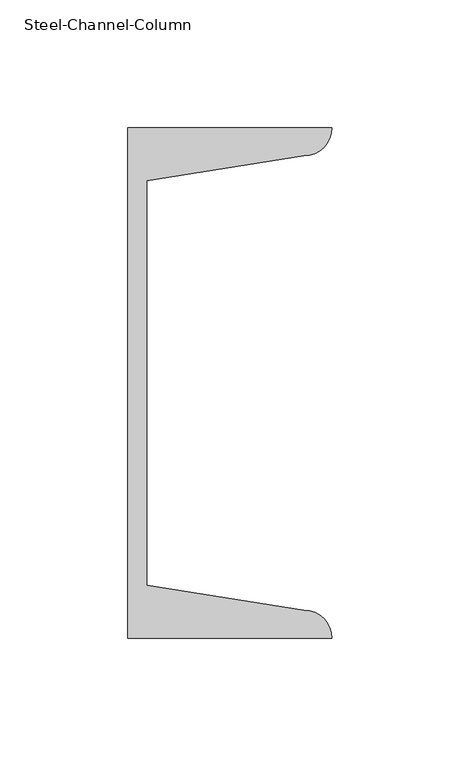
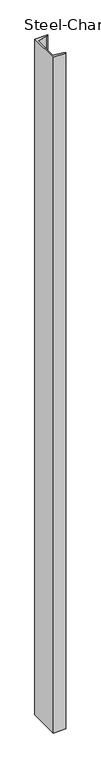
"""IFC4 building model written with IfcOpenShell, lengths in millimetres: column geometry, Steel-Channel-Column : CL126_C-200×80x7.5x11."""

import ifcopenshell
import ifcopenshell.guid

model = None  # the IFC model being written
_history = None  # IfcOwnerHistory: only IFC2X3 demands one
_inside = {}  # id of a spatial element -> (the spatial element, [elements in it])
_under = {}  # id of a project, library or spatial element -> (it, [spatial elements below it])
_declared = {}  # id of a project -> (the project, [libraries it declares])
_typed = {}  # id of a type object -> (the type object, [elements of that type])
_made_of = {}  # id of a material, layer set ... -> (it, [elements and type objects made of it])


def new_model(schema):
    """Start an empty IFC model of exactly this schema.

    Asked for "IFC4X3", IfcOpenShell would pick the latest addendum, in which some entities
    have other attributes; the version numbers below select the first issue.
    IFC2X3 requires an IfcOwnerHistory on every rooted entity: one is made here for all.
    """
    global model, _history
    if schema == "IFC4X3":
        model = ifcopenshell.file(schema_version=(4, 3, 0, 0))
    else:
        model = ifcopenshell.file(schema=schema)
    _inside.clear()
    _under.clear()
    _declared.clear()
    _typed.clear()
    _made_of.clear()
    _history = None
    if model.schema == "IFC2X3":
        org = make("IfcOrganization", Name="unknown")
        user = make(
            "IfcPersonAndOrganization",
            ThePerson=make("IfcPerson", FamilyName="unknown"),
            TheOrganization=org,
        )
        app = make(
            "IfcApplication",
            ApplicationDeveloper=org,
            Version="unknown",
            ApplicationFullName="unknown",
            ApplicationIdentifier="unknown",
        )
        _history = make(
            "IfcOwnerHistory",
            OwningUser=user,
            OwningApplication=app,
            ChangeAction="ADDED",
            CreationDate=0,
        )
    return model


def make(cls, **values):
    """One entity of the class cls with the attributes given. An attribute that is None is left unset."""
    return model.create_entity(
        cls, **{name: value for name, value in values.items() if value is not None}
    )


def rooted(cls, **values):
    """An entity with a GlobalId (a new one), such as an element, a storey or a relation."""
    return make(cls, GlobalId=ifcopenshell.guid.new(), OwnerHistory=_history, **values)


def si_unit(unit_type, name, prefix=None):
    """IfcSIUnit, for example si_unit("LENGTHUNIT", "METRE", prefix="MILLI")."""
    return make("IfcSIUnit", UnitType=unit_type, Prefix=prefix, Name=name)


def assignment(units):
    """IfcUnitAssignment: the units of a project."""
    return None if units is None else make("IfcUnitAssignment", Units=units)


def point(xyz):
    """IfcCartesianPoint."""
    return None if xyz is None else make("IfcCartesianPoint", Coordinates=xyz)


def direction(xyz):
    """IfcDirection."""
    return None if xyz is None else make("IfcDirection", DirectionRatios=xyz)


def frame(location, z_axis=None, x_axis=None):
    """IfcAxis2Placement3D, a coordinate frame: its origin and axes. An axis left out is left unset."""
    return make(
        "IfcAxis2Placement3D",
        Location=point(location),
        Axis=direction(z_axis),
        RefDirection=direction(x_axis),
    )


def frame_2d(location, x_axis=None):
    """IfcAxis2Placement2D, a coordinate frame in the plane: its origin and x axis."""
    return make(
        "IfcAxis2Placement2D", Location=point(location), RefDirection=direction(x_axis)
    )


def origin():
    """The frame at (0, 0, 0) with its axes left unset."""
    return frame((0.0, 0.0, 0.0))


def origin_with_axes():
    """The frame at (0, 0, 0) with the z axis (0, 0, 1) and the x axis (1, 0, 0) written out."""
    return frame((0.0, 0.0, 0.0), z_axis=(0.0, 0.0, 1.0), x_axis=(1.0, 0.0, 0.0))


def place(relative_to, where):
    """IfcLocalPlacement: puts the frame where relative to a parent placement (None: the world)."""
    return make(
        "IfcLocalPlacement", PlacementRelTo=relative_to, RelativePlacement=where
    )


def context(
    kind, dimensions, precision=None, world=None, true_north=None, identifier=None
):
    """IfcGeometricRepresentationContext, for example the 3D "Model" context."""
    return make(
        "IfcGeometricRepresentationContext",
        ContextIdentifier=identifier,
        ContextType=kind,
        CoordinateSpaceDimension=dimensions,
        Precision=precision,
        WorldCoordinateSystem=world,
        TrueNorth=true_north,
    )


def project(units=None, contexts=None):
    """IfcProject with its units and contexts."""
    return rooted(
        "IfcProject",
        Name="project",
        RepresentationContexts=contexts,
        UnitsInContext=assignment(units),
    )


def spatial(cls, under=None, at=None, **own):
    """A site, building, storey or space (cls), placed at a placement, below another one or the project."""
    s = rooted(cls, ObjectPlacement=at, **own)
    if under is not None:
        _under.setdefault(under.id(), (under, []))[1].append(s)
    return s


def polyline(points):
    """IfcPolyline through the points."""
    return make("IfcPolyline", Points=[point(p) for p in points])


def circle_curve(where, radius):
    """IfcCircle in the frame where."""
    return make("IfcCircle", Position=where, Radius=radius)


def trimmed(basis, trim1, trim2, sense, master):
    """IfcTrimmedCurve: the piece of a basis curve between two trims."""
    return make(
        "IfcTrimmedCurve",
        BasisCurve=basis,
        Trim1=trim1,
        Trim2=trim2,
        SenseAgreement=sense,
        MasterRepresentation=master,
    )


def segment(curve, same_sense, transition):
    """IfcCompositeCurveSegment."""
    return make(
        "IfcCompositeCurveSegment",
        Transition=transition,
        SameSense=same_sense,
        ParentCurve=curve,
    )


def composite_curve(segments, self_intersect=None):
    """IfcCompositeCurve: segments joined end to end."""
    return make("IfcCompositeCurve", Segments=segments, SelfIntersect=self_intersect)


def outline(outer, holes=None, kind="AREA"):
    """IfcArbitraryClosedProfileDef: a profile drawn as a closed curve; with holes, ...WithVoids."""
    if holes is None:
        return make("IfcArbitraryClosedProfileDef", ProfileType=kind, OuterCurve=outer)
    return make(
        "IfcArbitraryProfileDefWithVoids",
        ProfileType=kind,
        OuterCurve=outer,
        InnerCurves=holes,
    )


def extrude(swept, where, along, depth):
    """IfcExtrudedAreaSolid: the profile swept, set in the frame where, extruded along a direction by depth."""
    return make(
        "IfcExtrudedAreaSolid",
        SweptArea=swept,
        Position=where,
        ExtrudedDirection=direction(along),
        Depth=depth,
    )


def shape(context_of_items, identifier, shape_type, items):
    """IfcShapeRepresentation: the items that make up one representation, for example the "Body"."""
    return make(
        "IfcShapeRepresentation",
        ContextOfItems=context_of_items,
        RepresentationIdentifier=identifier,
        RepresentationType=shape_type,
        Items=items,
    )


def source(mapping_origin, context_of_items, identifier, shape_type, items):
    """IfcRepresentationMap: a shape defined once, which mapped items show again and again."""
    return make(
        "IfcRepresentationMap",
        MappingOrigin=mapping_origin,
        MappedRepresentation=shape(context_of_items, identifier, shape_type, items),
    )


def transform(
    local_origin,
    x_axis=None,
    y_axis=None,
    z_axis=None,
    scale=None,
    scale2=None,
    scale3=None,
    uniform=True,
):
    """IfcCartesianTransformationOperator3D, or its non-uniform kind. x_axis, y_axis, z_axis: its Axis1, 2, 3."""
    if uniform:
        return make(
            "IfcCartesianTransformationOperator3D",
            Axis1=direction(x_axis),
            Axis2=direction(y_axis),
            LocalOrigin=point(local_origin),
            Scale=scale,
            Axis3=direction(z_axis),
        )
    return make(
        "IfcCartesianTransformationOperator3DnonUniform",
        Axis1=direction(x_axis),
        Axis2=direction(y_axis),
        LocalOrigin=point(local_origin),
        Scale=scale,
        Axis3=direction(z_axis),
        Scale2=scale2,
        Scale3=scale3,
    )


def mapped(mapping_source, mapping_target):
    """IfcMappedItem: shows the shape of a source again, moved by a transform."""
    return make(
        "IfcMappedItem", MappingSource=mapping_source, MappingTarget=mapping_target
    )


def made_of(thing, what):
    """Note that an element or type object is made of a material, layer set ...; save() writes the relation."""
    if what is not None:
        _made_of.setdefault(what.id(), (what, []))[1].append(thing)
    return thing


def element(
    cls,
    number,
    at=None,
    inside=None,
    cuts=None,
    type_object=None,
    material=None,
    context=None,
    identifier="Body",
    shape_type=None,
    held_by="IfcProductDefinitionShape",
    body=None,
    shapes=None,
    **own,
):
    """One element of the class cls, such as IfcWall. Its Tag is "e" and its number.

    at: its placement. inside: the storey or other place that contains it. cuts: it is an
    opening in that element (IfcRelVoidsElement). A single representation is given by context,
    identifier, shape_type and body (its items); several are given by shapes. held_by: the class
    of the entity that holds the representations. save() writes the other relations.
    """
    e = rooted(cls, Tag="e%d" % number, ObjectPlacement=at, **own)
    if body is not None:
        shapes = [shape(context, identifier, shape_type, body)]
    if shapes is not None:
        e.Representation = make(held_by, Representations=shapes)
    if inside is not None:
        _inside.setdefault(inside.id(), (inside, []))[1].append(e)
    if cuts is not None:
        rooted(
            "IfcRelVoidsElement", RelatingBuildingElement=cuts, RelatedOpeningElement=e
        )
    if type_object is not None:
        _typed.setdefault(type_object.id(), (type_object, []))[1].append(e)
    return made_of(e, material)


def aggregate(whole, parts):
    """IfcRelAggregates: a whole, such as a stair, and the parts it consists of."""
    return rooted("IfcRelAggregates", RelatingObject=whole, RelatedObjects=parts)


def save(model, path):
    """Write the relations noted so far, then the file.

    IfcRelAggregates (storeys below a building ...), IfcRelContainedInSpatialStructure (elements
    in a storey), IfcRelDefinesByType, IfcRelAssociatesMaterial and IfcRelDeclares: one each for
    every whole, place, type object, material and project.
    """
    for whole, parts in _under.values():
        aggregate(whole, parts)
    for where, things in _inside.values():
        rooted(
            "IfcRelContainedInSpatialStructure",
            RelatedElements=things,
            RelatingStructure=where,
        )
    for kind, things in _typed.values():
        rooted("IfcRelDefinesByType", RelatedObjects=things, RelatingType=kind)
    for what, things in _made_of.values():
        rooted("IfcRelAssociatesMaterial", RelatedObjects=things, RelatingMaterial=what)
    for by, libraries in _declared.values():
        rooted("IfcRelDeclares", RelatingContext=by, RelatedDefinitions=libraries)
    model.write(path)


def steel_channel_column_de75dd10(model_context):
    return source(origin(), model_context, "Body", "SweptSolid", [
        extrude(outline(composite_curve([segment(polyline([(-22.1, 100.0), (57.9, 100.0)]), True, "CONTINUOUS"), segment(trimmed(circle_curve(frame_2d((46.9, 100.0)), 11.0), [point((57.9, 100.0))], [point((46.9, 89.0))], False, "CARTESIAN"), True, "CONTINUOUS"), segment(polyline([(46.9, 89.0), (-14.6, 79.2593569), (-14.6, -79.2593569), (46.9, -89.0)]), True, "CONTINUOUS"), segment(trimmed(circle_curve(frame_2d((46.9, -100.0)), 11.0), [point((46.9, -89.0))], [point((57.9, -100.0))], False, "CARTESIAN"), True, "CONTINUOUS"), segment(polyline([(57.9, -100.0), (-22.1, -100.0), (-22.1, 100.0)]), True, "CONTINUOUS")], self_intersect=False)), origin_with_axes(), (0.0, 0.0, 1.0), 4500.0),
    ])


if __name__ == "__main__":
    model = new_model("IFC4")
    model_context = context("Model", 3, world=origin())
    ifc_project = project(units=[si_unit("LENGTHUNIT", "METRE", prefix="MILLI")], contexts=[model_context])
    site = spatial("IfcSite", under=ifc_project)
    building = spatial("IfcBuilding", under=site)
    placement = place(None, origin())
    steel_channel_column_shape = steel_channel_column_de75dd10(model_context)
    element("IfcColumn", 1, ObjectType="Steel-Channel-Column : CL126_C-200×80x7.5x11", at=placement, inside=building, context=model_context, shape_type="MappedRepresentation", body=[
        mapped(steel_channel_column_shape, transform((0.0, 0.0, 0.0), x_axis=(1.0, 0.0, 0.0), y_axis=(0.0, 1.0, 0.0), z_axis=(0.0, 0.0, 1.0))),
    ])
    save(model, "model.ifc")

# Revit data of these elements
# Type "Steel-Channel-Column : CL126_C-200×80x7.5x11"
#   Assembly Code = "B10"
#   x = 22.1 mm
#   Section Area = 31.33 cm²
#   Mass per Unit Length = 24.60 kg/m
#   bf = 80 mm
#   d = 200 mm
#   tf = 11 mm
#   tw = 7.5 mm
#   hec_material4 [instance default] = none
#   hec_material3 [instance default] = none
#   hec_material2 [instance default] = none
#   hec_material1 [instance default] = none
#   Structural Material [instance default] = Steel, 45-345
# Element 1 (IfcColumn, "Steel-Channel-Column : CL126_C-200×80x7.5x11")
#   Materials on its faces: "Steel, 45-345"
# Materials
#   "Steel, 45-345": class "Metal", colour RGB 189 187 185, transparency 0, Description = "Steel 345 MPa", Cost = 0
